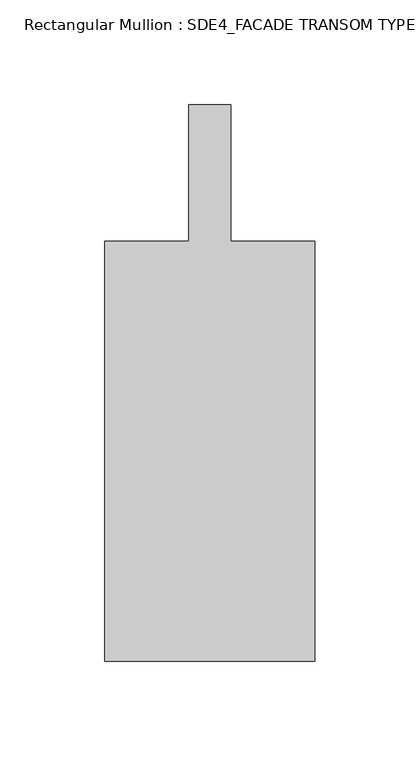
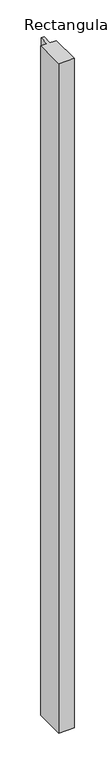
"""IFC4 building model written with IfcOpenShell, lengths in millimetres: member geometry, Rectangular Mullion : SDE4_FACADE TRANSOM TYPE 2."""

from ifc_helpers import new_model, si_unit, frame, origin, place, context, project, spatial, polyline, outline, extrude, source, transform, mapped, element, save


def rectangular_mullion_sde4_facade_transom_type_2_6ff46f1a(model_context):
    return source(origin(), model_context, "Body", "SweptSolid", [
        extrude(outline(polyline([(50.0, -132.5), (-50.0, -132.5), (-50.0, 67.5), (-10.0, 67.5), (-10.0, 132.5), (10.0, 132.5), (10.0, 67.5), (50.0, 67.5), (50.0, -132.5)])), frame((0.0, 0.0, -4578.0), z_axis=(0.0, 0.0, 1.0), x_axis=(1.0, 0.0, 0.0)), (0.0, 0.0, 1.0), 4578.0),
    ])


if __name__ == "__main__":
    model = new_model("IFC4")
    model_context = context("Model", 3, world=origin())
    ifc_project = project(units=[si_unit("LENGTHUNIT", "METRE", prefix="MILLI")], contexts=[model_context])
    site = spatial("IfcSite", under=ifc_project)
    building = spatial("IfcBuilding", under=site)
    placement = place(None, origin())
    rectangular_mullion_sde4_facade_transom_type_2_shape = rectangular_mullion_sde4_facade_transom_type_2_6ff46f1a(model_context)
    element("IfcMember", 1, ObjectType="Rectangular Mullion : SDE4_FACADE TRANSOM TYPE 2", at=placement, inside=building, context=model_context, shape_type="MappedRepresentation", body=[
        mapped(rectangular_mullion_sde4_facade_transom_type_2_shape, transform((0.0, 0.0, 0.0), x_axis=(1.0, 0.0, 0.0), y_axis=(0.0, 1.0, 0.0), z_axis=(0.0, 0.0, 1.0))),
    ])
    save(model, "model.ifc")

# Revit data of these elements
# Type "Rectangular Mullion : SDE4_FACADE TRANSOM TYPE 2"
#   built-in parameter 1007322 = 0.869423 (stored number, unit not read)
#   built-in parameter 1007321 = 0.164042 (stored number, unit not read)
#   built-in parameter 1007320 = 0.164042 (stored number, unit not read)
